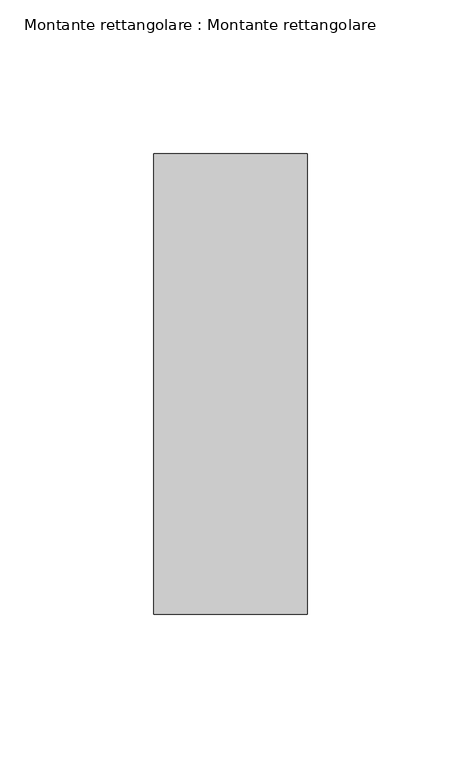
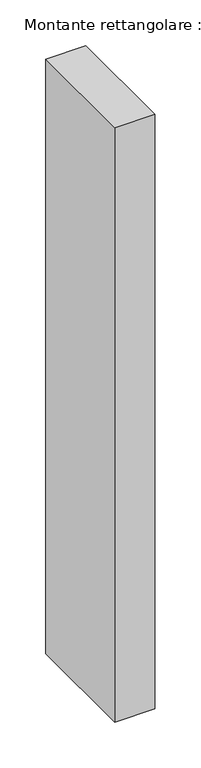
"""IFC4 building model written with IfcOpenShell, lengths in millimetres: member geometry, Montante rettangolare : Montante rettangolare."""

from ifc_helpers import new_model, si_unit, frame, origin, place, context, project, spatial, polyline, outline, extrude, source, transform, mapped, element, save


def montante_rettangolare_montante_rettangolare_0b28999b(model_context):
    return source(origin(), model_context, "Body", "SweptSolid", [
        extrude(outline(polyline([(25.0, 75.0), (25.0, -75.0), (-25.0, -75.0), (-25.0, 75.0), (25.0, 75.0)])), frame((0.0, 0.0, -790.0), z_axis=(0.0, 0.0, 1.0), x_axis=(1.0, 0.0, 0.0)), (0.0, 0.0, 1.0), 790.0),
    ])


if __name__ == "__main__":
    model = new_model("IFC4")
    model_context = context("Model", 3, world=origin())
    ifc_project = project(units=[si_unit("LENGTHUNIT", "METRE", prefix="MILLI")], contexts=[model_context])
    site = spatial("IfcSite", under=ifc_project)
    building = spatial("IfcBuilding", under=site)
    placement = place(None, origin())
    montante_rettangolare_montante_rettangolare_shape = montante_rettangolare_montante_rettangolare_0b28999b(model_context)
    element("IfcMember", 1, ObjectType="Montante rettangolare : Montante rettangolare", at=placement, inside=building, context=model_context, shape_type="MappedRepresentation", body=[
        mapped(montante_rettangolare_montante_rettangolare_shape, transform((0.0, 0.0, 0.0), x_axis=(1.0, 0.0, 0.0), y_axis=(0.0, 1.0, 0.0), z_axis=(0.0, 0.0, 1.0))),
    ])
    save(model, "model.ifc")

# Revit data of these elements
# Type "Montante rettangolare : Montante rettangolare"
#   built-in parameter 1007304 = 0.492126 (stored number, unit not read)
#   built-in parameter 1007301 = 0.082021 (stored number, unit not read)
#   built-in parameter 1007300 = 0.082021 (stored number, unit not read)
# Element 1 (IfcMember, "Montante rettangolare : Montante rettangolare")
#   Materials on its faces: "Acciaio"
# Materials
#   "Acciaio": class "Metallo", colour RGB 247 247 247, transparency 0, Description = "Acciaio, finitura zigrinata", Cost = 0
